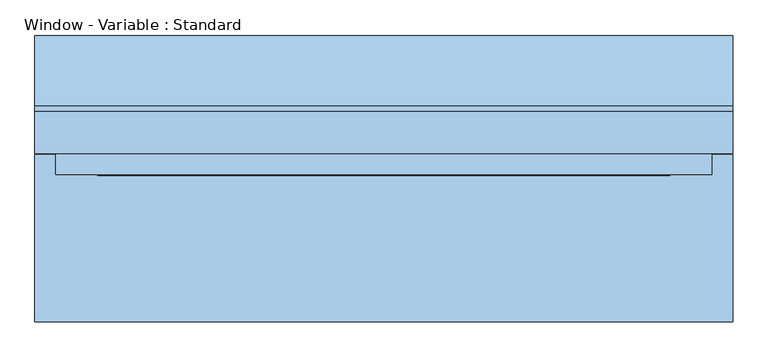
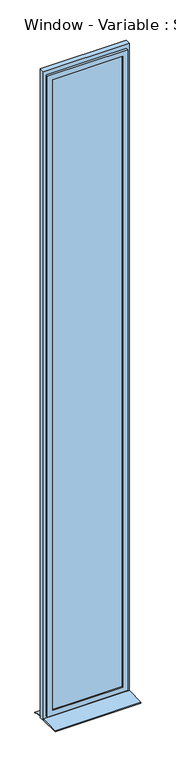
"""IFC4 building model written with IfcOpenShell, lengths in millimetres: window geometry, Window - Variable : Standard."""

from ifc_helpers import new_model, si_unit, frame, origin, place, context, project, spatial, polyline, outline, extrude, faceted_brep, source, transform, mapped, element, save


def window_variable_standard_5cf830ff(model_context):
    return source(origin(), model_context, "Body", "SolidModel", [
        extrude(outline(polyline([(9000.0, 500.0), (9000.0, -500.0), (1000.0, -500.0), (1000.0, 500.0), (9000.0, 500.0)]), holes=[polyline([(8920.0, 440.0), (1080.0, 440.0), (1080.0, -440.0), (8920.0, -440.0), (8920.0, 440.0)])]), frame((0.0, 35.0, 0.0), z_axis=(0.0, 1.0, 0.0), x_axis=(0.0, 0.0, 1.0)), (0.0, 0.0, 1.0), 60.0),
        faceted_brep([(470.0, 35.0, 8950.0), (470.0, 5.0, 8950.0), (470.0, 5.0, 1050.0), (470.0, 35.0, 1050.0), (-470.0, 5.0, 8950.0), (-470.0, 5.0, 1050.0), (410.0, 5.0, 1110.0), (-410.0, 5.0, 1110.0), (-410.0, 5.0, 8890.0), (410.0, 5.0, 8890.0), (-470.0, 35.0, 1050.0), (-470.0, 35.0, 8950.0), (440.0, 35.0, 8920.0), (-440.0, 35.0, 8920.0), (-440.0, 35.0, 1080.0), (440.0, 35.0, 1080.0), (440.0, 65.0, 8920.0), (440.0, 65.0, 1080.0), (-440.0, 65.0, 1080.0), (-440.0, 65.0, 8920.0), (410.0, 65.0, 8890.0), (-410.0, 65.0, 8890.0), (-410.0, 65.0, 1110.0), (410.0, 65.0, 1110.0)], [[[0, 1, 2, 3]], [[1, 4, 5, 2], [6, 7, 8, 9]], [[3, 2, 5, 10]], [[3, 10, 11, 0], [12, 13, 14, 15]], [[16, 12, 15, 17]], [[17, 15, 14, 18]], [[17, 18, 19, 16], [20, 21, 22, 23]], [[9, 20, 23, 6]], [[6, 23, 22, 7]], [[10, 5, 4, 11]], [[18, 14, 13, 19]], [[7, 22, 21, 8]], [[11, 4, 1, 0]], [[19, 13, 12, 16]], [[8, 21, 20, 9]]]),
        extrude(outline(polyline([(-500.0, -205.0), (-500.0, 35.0), (500.0, 35.0), (500.0, -205.0), (-500.0, -205.0)])), frame((0.0, 0.0, 1005.0), z_axis=(0.0, 0.0, 1.0), x_axis=(1.0, 0.0, 0.0)), (0.0, 0.0, 1.0), 15.0),
        extrude(outline(polyline([(105.0221543, 1020.0), (205.0, 1000.0), (205.0, 990.0), (203.0, 990.0), (203.0, 998.3604634), (104.8240723, 1018.0), (95.0, 1018.0), (95.0, 1020.0), (105.0221543, 1020.0)])), frame((-500.0, 0.0, 0.0), z_axis=(1.0, 0.0, 0.0), x_axis=(0.0, 1.0, 0.0)), (0.0, 0.0, 1.0), 1000.0),
        extrude(outline(polyline([(410.0, 20.0), (-410.0, 20.0), (-410.0, 50.0), (410.0, 50.0), (410.0, 20.0)])), frame((0.0, 0.0, 1110.0), z_axis=(0.0, 0.0, 1.0), x_axis=(1.0, 0.0, 0.0)), (0.0, 0.0, 1.0), 7780.0),
    ])


if __name__ == "__main__":
    model = new_model("IFC4")
    model_context = context("Model", 3, world=origin())
    ifc_project = project(units=[si_unit("LENGTHUNIT", "METRE", prefix="MILLI")], contexts=[model_context])
    site = spatial("IfcSite", under=ifc_project)
    building = spatial("IfcBuilding", under=site)
    placement = place(None, origin())
    window_variable_standard_shape = window_variable_standard_5cf830ff(model_context)
    element("IfcWindow", 1, ObjectType="Window - Variable : Standard", at=placement, inside=building, context=model_context, shape_type="MappedRepresentation", body=[
        mapped(window_variable_standard_shape, transform((0.0, 0.0, 0.0), x_axis=(1.0, 0.0, 0.0), y_axis=(0.0, 1.0, 0.0), z_axis=(0.0, 0.0, 1.0))),
    ])
    save(model, "model.ifc")

# Revit data of these elements
# Type "Window - Variable : Standard"
#   Type Mark = "19"
#   Operation = "SinglePanel"
#   Keynote = "16.05.01"
#   Analytic Construction = "<None>"
#   Rough Width [instance default] = 1.010 m
#   Rough Height [instance default] = 1.010 m
#   Frame Depth = 0.060 m
#   Frame Height Bottom = 0.080 m
#   Frame Height Top = 0.080 m
#   Frame Width = 0.060 m
#   Height [instance default] = 1.010 m
#   Window Inset = 0.060 m
#   Window Width = 0.060 m
#   Instalation Depth [instance default] = 0.080 m
#   Width [instance default] = 1.010 m
#   Folding Wing [instance default] = no
#   Oppening Direction Vertical [instance default] = yes
#   Oppening Direction Visibility [instance default] = no
#   Casement [instance default] = yes
#   Frame [instance default] = none
#   Glas [instance default] = none
#   Window [instance default] = none
#   Windowsill Inside [instance default] = none
#   Windowsill Outside [instance default] = none
#   Wall Closure = (empty or 0)
#   Assembly Code = ""
# Element 1 (IfcWindow, "Window - Variable : Standard")
#   Rough Width = 1.000 m
#   Rough Height = 8.000 m
#   Height = 8.000 m
#   Width = 1.000 m
#   Materials on its faces: "Plastic - White", "Metal _ Aluminium", "Wood - Birch", "Glass"
# Materials
#   "Plastic - White": class "Kunststoff", colour RGB 249 249 249, transparency 0
#   "Metal _ Aluminium": class "Metall", colour RGB 247 247 247, transparency 0
#   "Wood - Birch": class "Holz", colour RGB 213 164 103, transparency 0
#   "Glass": class "Glass", colour RGB 0 128 192, transparency 0.9
